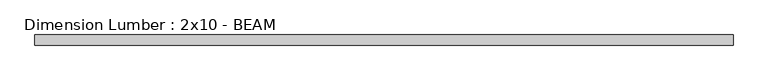
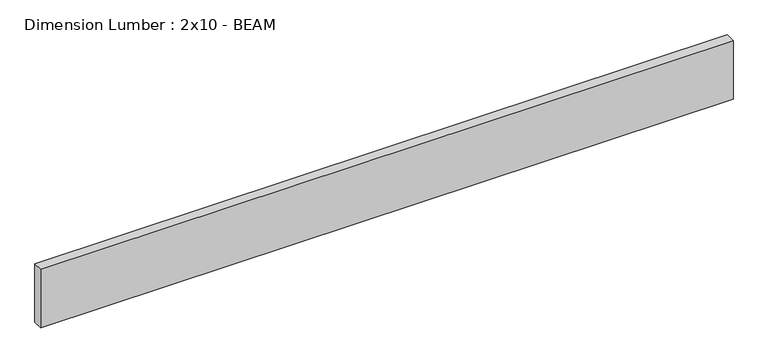
"""IFC4 building model written with IfcOpenShell, lengths in millimetres: beam geometry, Dimension Lumber : 2x10 - BEAM."""

import ifcopenshell
import ifcopenshell.guid

model = None  # the IFC model being written
_history = None  # IfcOwnerHistory: only IFC2X3 demands one
_inside = {}  # id of a spatial element -> (the spatial element, [elements in it])
_under = {}  # id of a project, library or spatial element -> (it, [spatial elements below it])
_declared = {}  # id of a project -> (the project, [libraries it declares])
_typed = {}  # id of a type object -> (the type object, [elements of that type])
_made_of = {}  # id of a material, layer set ... -> (it, [elements and type objects made of it])


def new_model(schema):
    """Start an empty IFC model of exactly this schema.

    Asked for "IFC4X3", IfcOpenShell would pick the latest addendum, in which some entities
    have other attributes; the version numbers below select the first issue.
    IFC2X3 requires an IfcOwnerHistory on every rooted entity: one is made here for all.
    """
    global model, _history
    if schema == "IFC4X3":
        model = ifcopenshell.file(schema_version=(4, 3, 0, 0))
    else:
        model = ifcopenshell.file(schema=schema)
    _inside.clear()
    _under.clear()
    _declared.clear()
    _typed.clear()
    _made_of.clear()
    _history = None
    if model.schema == "IFC2X3":
        org = make("IfcOrganization", Name="unknown")
        user = make(
            "IfcPersonAndOrganization",
            ThePerson=make("IfcPerson", FamilyName="unknown"),
            TheOrganization=org,
        )
        app = make(
            "IfcApplication",
            ApplicationDeveloper=org,
            Version="unknown",
            ApplicationFullName="unknown",
            ApplicationIdentifier="unknown",
        )
        _history = make(
            "IfcOwnerHistory",
            OwningUser=user,
            OwningApplication=app,
            ChangeAction="ADDED",
            CreationDate=0,
        )
    return model


def make(cls, **values):
    """One entity of the class cls with the attributes given. An attribute that is None is left unset."""
    return model.create_entity(
        cls, **{name: value for name, value in values.items() if value is not None}
    )


def rooted(cls, **values):
    """An entity with a GlobalId (a new one), such as an element, a storey or a relation."""
    return make(cls, GlobalId=ifcopenshell.guid.new(), OwnerHistory=_history, **values)


def si_unit(unit_type, name, prefix=None):
    """IfcSIUnit, for example si_unit("LENGTHUNIT", "METRE", prefix="MILLI")."""
    return make("IfcSIUnit", UnitType=unit_type, Prefix=prefix, Name=name)


def assignment(units):
    """IfcUnitAssignment: the units of a project."""
    return None if units is None else make("IfcUnitAssignment", Units=units)


def point(xyz):
    """IfcCartesianPoint."""
    return None if xyz is None else make("IfcCartesianPoint", Coordinates=xyz)


def direction(xyz):
    """IfcDirection."""
    return None if xyz is None else make("IfcDirection", DirectionRatios=xyz)


def frame(location, z_axis=None, x_axis=None):
    """IfcAxis2Placement3D, a coordinate frame: its origin and axes. An axis left out is left unset."""
    return make(
        "IfcAxis2Placement3D",
        Location=point(location),
        Axis=direction(z_axis),
        RefDirection=direction(x_axis),
    )


def origin():
    """The frame at (0, 0, 0) with its axes left unset."""
    return frame((0.0, 0.0, 0.0))


def place(relative_to, where):
    """IfcLocalPlacement: puts the frame where relative to a parent placement (None: the world)."""
    return make(
        "IfcLocalPlacement", PlacementRelTo=relative_to, RelativePlacement=where
    )


def context(
    kind, dimensions, precision=None, world=None, true_north=None, identifier=None
):
    """IfcGeometricRepresentationContext, for example the 3D "Model" context."""
    return make(
        "IfcGeometricRepresentationContext",
        ContextIdentifier=identifier,
        ContextType=kind,
        CoordinateSpaceDimension=dimensions,
        Precision=precision,
        WorldCoordinateSystem=world,
        TrueNorth=true_north,
    )


def project(units=None, contexts=None):
    """IfcProject with its units and contexts."""
    return rooted(
        "IfcProject",
        Name="project",
        RepresentationContexts=contexts,
        UnitsInContext=assignment(units),
    )


def spatial(cls, under=None, at=None, **own):
    """A site, building, storey or space (cls), placed at a placement, below another one or the project."""
    s = rooted(cls, ObjectPlacement=at, **own)
    if under is not None:
        _under.setdefault(under.id(), (under, []))[1].append(s)
    return s


def polyline(points):
    """IfcPolyline through the points."""
    return make("IfcPolyline", Points=[point(p) for p in points])


def outline(outer, holes=None, kind="AREA"):
    """IfcArbitraryClosedProfileDef: a profile drawn as a closed curve; with holes, ...WithVoids."""
    if holes is None:
        return make("IfcArbitraryClosedProfileDef", ProfileType=kind, OuterCurve=outer)
    return make(
        "IfcArbitraryProfileDefWithVoids",
        ProfileType=kind,
        OuterCurve=outer,
        InnerCurves=holes,
    )


def extrude(swept, where, along, depth):
    """IfcExtrudedAreaSolid: the profile swept, set in the frame where, extruded along a direction by depth."""
    return make(
        "IfcExtrudedAreaSolid",
        SweptArea=swept,
        Position=where,
        ExtrudedDirection=direction(along),
        Depth=depth,
    )


def shape(context_of_items, identifier, shape_type, items):
    """IfcShapeRepresentation: the items that make up one representation, for example the "Body"."""
    return make(
        "IfcShapeRepresentation",
        ContextOfItems=context_of_items,
        RepresentationIdentifier=identifier,
        RepresentationType=shape_type,
        Items=items,
    )


def source(mapping_origin, context_of_items, identifier, shape_type, items):
    """IfcRepresentationMap: a shape defined once, which mapped items show again and again."""
    return make(
        "IfcRepresentationMap",
        MappingOrigin=mapping_origin,
        MappedRepresentation=shape(context_of_items, identifier, shape_type, items),
    )


def transform(
    local_origin,
    x_axis=None,
    y_axis=None,
    z_axis=None,
    scale=None,
    scale2=None,
    scale3=None,
    uniform=True,
):
    """IfcCartesianTransformationOperator3D, or its non-uniform kind. x_axis, y_axis, z_axis: its Axis1, 2, 3."""
    if uniform:
        return make(
            "IfcCartesianTransformationOperator3D",
            Axis1=direction(x_axis),
            Axis2=direction(y_axis),
            LocalOrigin=point(local_origin),
            Scale=scale,
            Axis3=direction(z_axis),
        )
    return make(
        "IfcCartesianTransformationOperator3DnonUniform",
        Axis1=direction(x_axis),
        Axis2=direction(y_axis),
        LocalOrigin=point(local_origin),
        Scale=scale,
        Axis3=direction(z_axis),
        Scale2=scale2,
        Scale3=scale3,
    )


def mapped(mapping_source, mapping_target):
    """IfcMappedItem: shows the shape of a source again, moved by a transform."""
    return make(
        "IfcMappedItem", MappingSource=mapping_source, MappingTarget=mapping_target
    )


def made_of(thing, what):
    """Note that an element or type object is made of a material, layer set ...; save() writes the relation."""
    if what is not None:
        _made_of.setdefault(what.id(), (what, []))[1].append(thing)
    return thing


def element(
    cls,
    number,
    at=None,
    inside=None,
    cuts=None,
    type_object=None,
    material=None,
    context=None,
    identifier="Body",
    shape_type=None,
    held_by="IfcProductDefinitionShape",
    body=None,
    shapes=None,
    **own,
):
    """One element of the class cls, such as IfcWall. Its Tag is "e" and its number.

    at: its placement. inside: the storey or other place that contains it. cuts: it is an
    opening in that element (IfcRelVoidsElement). A single representation is given by context,
    identifier, shape_type and body (its items); several are given by shapes. held_by: the class
    of the entity that holds the representations. save() writes the other relations.
    """
    e = rooted(cls, Tag="e%d" % number, ObjectPlacement=at, **own)
    if body is not None:
        shapes = [shape(context, identifier, shape_type, body)]
    if shapes is not None:
        e.Representation = make(held_by, Representations=shapes)
    if inside is not None:
        _inside.setdefault(inside.id(), (inside, []))[1].append(e)
    if cuts is not None:
        rooted(
            "IfcRelVoidsElement", RelatingBuildingElement=cuts, RelatedOpeningElement=e
        )
    if type_object is not None:
        _typed.setdefault(type_object.id(), (type_object, []))[1].append(e)
    return made_of(e, material)


def aggregate(whole, parts):
    """IfcRelAggregates: a whole, such as a stair, and the parts it consists of."""
    return rooted("IfcRelAggregates", RelatingObject=whole, RelatedObjects=parts)


def save(model, path):
    """Write the relations noted so far, then the file.

    IfcRelAggregates (storeys below a building ...), IfcRelContainedInSpatialStructure (elements
    in a storey), IfcRelDefinesByType, IfcRelAssociatesMaterial and IfcRelDeclares: one each for
    every whole, place, type object, material and project.
    """
    for whole, parts in _under.values():
        aggregate(whole, parts)
    for where, things in _inside.values():
        rooted(
            "IfcRelContainedInSpatialStructure",
            RelatedElements=things,
            RelatingStructure=where,
        )
    for kind, things in _typed.values():
        rooted("IfcRelDefinesByType", RelatedObjects=things, RelatingType=kind)
    for what, things in _made_of.values():
        rooted("IfcRelAssociatesMaterial", RelatedObjects=things, RelatingMaterial=what)
    for by, libraries in _declared.values():
        rooted("IfcRelDeclares", RelatingContext=by, RelatedDefinitions=libraries)
    model.write(path)


def dimension_lumber_2x10_beam_af6f43a0(model_context):
    return source(origin(), model_context, "Body", "SweptSolid", [
        extrude(outline(polyline([(1293.5856544, 19.05), (1293.5856544, -19.05), (-1334.8606544, -19.05), (-1334.8606544, 19.05), (1293.5856544, 19.05)])), frame((0.0, 0.0, -117.475), z_axis=(0.0, 0.0, 1.0), x_axis=(1.0, 0.0, 0.0)), (0.0, 0.0, 1.0), 234.95),
    ])


if __name__ == "__main__":
    model = new_model("IFC4")
    model_context = context("Model", 3, world=origin())
    ifc_project = project(units=[si_unit("LENGTHUNIT", "METRE", prefix="MILLI")], contexts=[model_context])
    site = spatial("IfcSite", under=ifc_project)
    building = spatial("IfcBuilding", under=site)
    placement = place(None, origin())
    dimension_lumber_2x10_beam_shape = dimension_lumber_2x10_beam_af6f43a0(model_context)
    element("IfcBeam", 1, ObjectType="Dimension Lumber : 2x10 - BEAM", at=placement, inside=building, context=model_context, shape_type="MappedRepresentation", body=[
        mapped(dimension_lumber_2x10_beam_shape, transform((0.0, 0.0, 0.0), x_axis=(1.0, 0.0, 0.0), y_axis=(0.0, 1.0, 0.0), z_axis=(0.0, 0.0, 1.0))),
    ])
    save(model, "model.ifc")

# Revit data of these elements
# Type "Dimension Lumber : 2x10 - BEAM"
#   Assembly Code = "B10"
#   A = 0.0755556 SF
#   Length [instance default] = 5' - 0"
#   b = 0' - 1 1/2"
#   d = 0' - 9 1/4"
#   Structural Material = (3) SISTERED 2X10s AT BEAM
# Element 1 (IfcBeam, "Dimension Lumber : 2x10 - BEAM")
#   Materials on its faces: "(3) SISTERED 2X10s AT BEAM"
# Materials
#   "(3) SISTERED 2X10s AT BEAM": class "Wood", colour RGB 234 198 147, transparency 0, Description = "Pinus Echinata", Cost = 0
